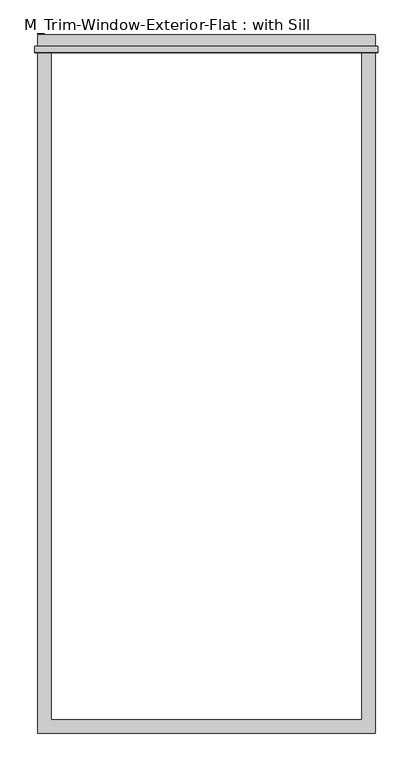
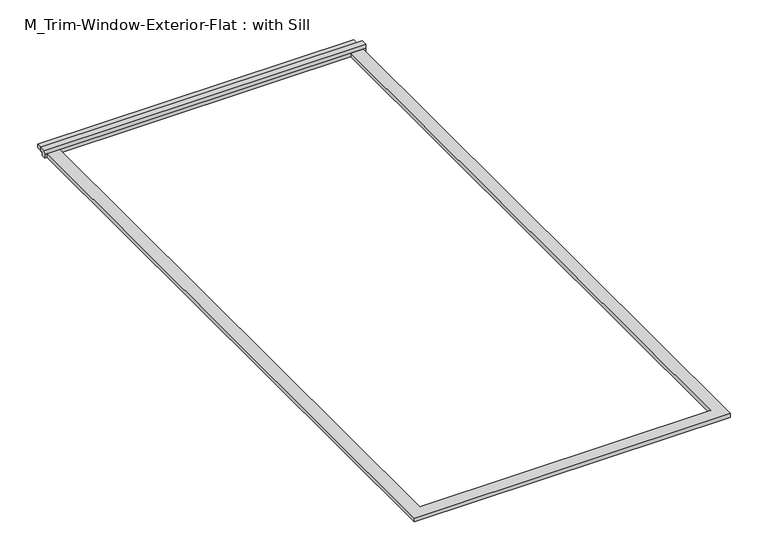
"""IFC4 building model written with IfcOpenShell, lengths in millimetres: proxy geometry, M_Trim-Window-Exterior-Flat : with Sill."""

import ifcopenshell
import ifcopenshell.guid

model = None  # the IFC model being written
_history = None  # IfcOwnerHistory: only IFC2X3 demands one
_inside = {}  # id of a spatial element -> (the spatial element, [elements in it])
_under = {}  # id of a project, library or spatial element -> (it, [spatial elements below it])
_declared = {}  # id of a project -> (the project, [libraries it declares])
_typed = {}  # id of a type object -> (the type object, [elements of that type])
_made_of = {}  # id of a material, layer set ... -> (it, [elements and type objects made of it])


def new_model(schema):
    """Start an empty IFC model of exactly this schema.

    Asked for "IFC4X3", IfcOpenShell would pick the latest addendum, in which some entities
    have other attributes; the version numbers below select the first issue.
    IFC2X3 requires an IfcOwnerHistory on every rooted entity: one is made here for all.
    """
    global model, _history
    if schema == "IFC4X3":
        model = ifcopenshell.file(schema_version=(4, 3, 0, 0))
    else:
        model = ifcopenshell.file(schema=schema)
    _inside.clear()
    _under.clear()
    _declared.clear()
    _typed.clear()
    _made_of.clear()
    _history = None
    if model.schema == "IFC2X3":
        org = make("IfcOrganization", Name="unknown")
        user = make(
            "IfcPersonAndOrganization",
            ThePerson=make("IfcPerson", FamilyName="unknown"),
            TheOrganization=org,
        )
        app = make(
            "IfcApplication",
            ApplicationDeveloper=org,
            Version="unknown",
            ApplicationFullName="unknown",
            ApplicationIdentifier="unknown",
        )
        _history = make(
            "IfcOwnerHistory",
            OwningUser=user,
            OwningApplication=app,
            ChangeAction="ADDED",
            CreationDate=0,
        )
    return model


def make(cls, **values):
    """One entity of the class cls with the attributes given. An attribute that is None is left unset."""
    return model.create_entity(
        cls, **{name: value for name, value in values.items() if value is not None}
    )


def rooted(cls, **values):
    """An entity with a GlobalId (a new one), such as an element, a storey or a relation."""
    return make(cls, GlobalId=ifcopenshell.guid.new(), OwnerHistory=_history, **values)


def si_unit(unit_type, name, prefix=None):
    """IfcSIUnit, for example si_unit("LENGTHUNIT", "METRE", prefix="MILLI")."""
    return make("IfcSIUnit", UnitType=unit_type, Prefix=prefix, Name=name)


def assignment(units):
    """IfcUnitAssignment: the units of a project."""
    return None if units is None else make("IfcUnitAssignment", Units=units)


def point(xyz):
    """IfcCartesianPoint."""
    return None if xyz is None else make("IfcCartesianPoint", Coordinates=xyz)


def direction(xyz):
    """IfcDirection."""
    return None if xyz is None else make("IfcDirection", DirectionRatios=xyz)


def frame(location, z_axis=None, x_axis=None):
    """IfcAxis2Placement3D, a coordinate frame: its origin and axes. An axis left out is left unset."""
    return make(
        "IfcAxis2Placement3D",
        Location=point(location),
        Axis=direction(z_axis),
        RefDirection=direction(x_axis),
    )


def origin():
    """The frame at (0, 0, 0) with its axes left unset."""
    return frame((0.0, 0.0, 0.0))


def origin_with_axes():
    """The frame at (0, 0, 0) with the z axis (0, 0, 1) and the x axis (1, 0, 0) written out."""
    return frame((0.0, 0.0, 0.0), z_axis=(0.0, 0.0, 1.0), x_axis=(1.0, 0.0, 0.0))


def place(relative_to, where):
    """IfcLocalPlacement: puts the frame where relative to a parent placement (None: the world)."""
    return make(
        "IfcLocalPlacement", PlacementRelTo=relative_to, RelativePlacement=where
    )


def context(
    kind, dimensions, precision=None, world=None, true_north=None, identifier=None
):
    """IfcGeometricRepresentationContext, for example the 3D "Model" context."""
    return make(
        "IfcGeometricRepresentationContext",
        ContextIdentifier=identifier,
        ContextType=kind,
        CoordinateSpaceDimension=dimensions,
        Precision=precision,
        WorldCoordinateSystem=world,
        TrueNorth=true_north,
    )


def project(units=None, contexts=None):
    """IfcProject with its units and contexts."""
    return rooted(
        "IfcProject",
        Name="project",
        RepresentationContexts=contexts,
        UnitsInContext=assignment(units),
    )


def spatial(cls, under=None, at=None, **own):
    """A site, building, storey or space (cls), placed at a placement, below another one or the project."""
    s = rooted(cls, ObjectPlacement=at, **own)
    if under is not None:
        _under.setdefault(under.id(), (under, []))[1].append(s)
    return s


def polyline(points):
    """IfcPolyline through the points."""
    return make("IfcPolyline", Points=[point(p) for p in points])


def outline(outer, holes=None, kind="AREA"):
    """IfcArbitraryClosedProfileDef: a profile drawn as a closed curve; with holes, ...WithVoids."""
    if holes is None:
        return make("IfcArbitraryClosedProfileDef", ProfileType=kind, OuterCurve=outer)
    return make(
        "IfcArbitraryProfileDefWithVoids",
        ProfileType=kind,
        OuterCurve=outer,
        InnerCurves=holes,
    )


def extrude(swept, where, along, depth):
    """IfcExtrudedAreaSolid: the profile swept, set in the frame where, extruded along a direction by depth."""
    return make(
        "IfcExtrudedAreaSolid",
        SweptArea=swept,
        Position=where,
        ExtrudedDirection=direction(along),
        Depth=depth,
    )


def shape(context_of_items, identifier, shape_type, items):
    """IfcShapeRepresentation: the items that make up one representation, for example the "Body"."""
    return make(
        "IfcShapeRepresentation",
        ContextOfItems=context_of_items,
        RepresentationIdentifier=identifier,
        RepresentationType=shape_type,
        Items=items,
    )


def source(mapping_origin, context_of_items, identifier, shape_type, items):
    """IfcRepresentationMap: a shape defined once, which mapped items show again and again."""
    return make(
        "IfcRepresentationMap",
        MappingOrigin=mapping_origin,
        MappedRepresentation=shape(context_of_items, identifier, shape_type, items),
    )


def transform(
    local_origin,
    x_axis=None,
    y_axis=None,
    z_axis=None,
    scale=None,
    scale2=None,
    scale3=None,
    uniform=True,
):
    """IfcCartesianTransformationOperator3D, or its non-uniform kind. x_axis, y_axis, z_axis: its Axis1, 2, 3."""
    if uniform:
        return make(
            "IfcCartesianTransformationOperator3D",
            Axis1=direction(x_axis),
            Axis2=direction(y_axis),
            LocalOrigin=point(local_origin),
            Scale=scale,
            Axis3=direction(z_axis),
        )
    return make(
        "IfcCartesianTransformationOperator3DnonUniform",
        Axis1=direction(x_axis),
        Axis2=direction(y_axis),
        LocalOrigin=point(local_origin),
        Scale=scale,
        Axis3=direction(z_axis),
        Scale2=scale2,
        Scale3=scale3,
    )


def mapped(mapping_source, mapping_target):
    """IfcMappedItem: shows the shape of a source again, moved by a transform."""
    return make(
        "IfcMappedItem", MappingSource=mapping_source, MappingTarget=mapping_target
    )


def made_of(thing, what):
    """Note that an element or type object is made of a material, layer set ...; save() writes the relation."""
    if what is not None:
        _made_of.setdefault(what.id(), (what, []))[1].append(thing)
    return thing


def element(
    cls,
    number,
    at=None,
    inside=None,
    cuts=None,
    type_object=None,
    material=None,
    context=None,
    identifier="Body",
    shape_type=None,
    held_by="IfcProductDefinitionShape",
    body=None,
    shapes=None,
    **own,
):
    """One element of the class cls, such as IfcWall. Its Tag is "e" and its number.

    at: its placement. inside: the storey or other place that contains it. cuts: it is an
    opening in that element (IfcRelVoidsElement). A single representation is given by context,
    identifier, shape_type and body (its items); several are given by shapes. held_by: the class
    of the entity that holds the representations. save() writes the other relations.
    """
    e = rooted(cls, Tag="e%d" % number, ObjectPlacement=at, **own)
    if body is not None:
        shapes = [shape(context, identifier, shape_type, body)]
    if shapes is not None:
        e.Representation = make(held_by, Representations=shapes)
    if inside is not None:
        _inside.setdefault(inside.id(), (inside, []))[1].append(e)
    if cuts is not None:
        rooted(
            "IfcRelVoidsElement", RelatingBuildingElement=cuts, RelatedOpeningElement=e
        )
    if type_object is not None:
        _typed.setdefault(type_object.id(), (type_object, []))[1].append(e)
    return made_of(e, material)


def aggregate(whole, parts):
    """IfcRelAggregates: a whole, such as a stair, and the parts it consists of."""
    return rooted("IfcRelAggregates", RelatingObject=whole, RelatedObjects=parts)


def save(model, path):
    """Write the relations noted so far, then the file.

    IfcRelAggregates (storeys below a building ...), IfcRelContainedInSpatialStructure (elements
    in a storey), IfcRelDefinesByType, IfcRelAssociatesMaterial and IfcRelDeclares: one each for
    every whole, place, type object, material and project.
    """
    for whole, parts in _under.values():
        aggregate(whole, parts)
    for where, things in _inside.values():
        rooted(
            "IfcRelContainedInSpatialStructure",
            RelatedElements=things,
            RelatingStructure=where,
        )
    for kind, things in _typed.values():
        rooted("IfcRelDefinesByType", RelatedObjects=things, RelatingType=kind)
    for what, things in _made_of.values():
        rooted("IfcRelAssociatesMaterial", RelatedObjects=things, RelatingMaterial=what)
    for by, libraries in _declared.values():
        rooted("IfcRelDeclares", RelatingContext=by, RelatedDefinitions=libraries)
    model.write(path)


def m_trim_window_exterior_flat_with_sill_53234c90(model_context):
    return source(origin(), model_context, "Body", "SweptSolid", [
        extrude(outline(polyline([(760.0, 3020.4323709), (-760.0, 3020.4323709), (-760.0, 3080.4323709), (760.0, 3080.4323709), (760.0, 3020.4323709)])), origin_with_axes(), (0.0, 0.0, 1.0), 19.05),
        extrude(outline(polyline([(3030.0, 38.1), (3030.0, 19.05), (3020.4323709, 19.05), (3020.4323709, 0.0), (3000.0, 0.0), (3000.0, 19.05), (3002.4580645, 38.1), (3030.0, 38.1)])), frame((-772.7, 0.0, 0.0), z_axis=(1.0, 0.0, 0.0), x_axis=(0.0, 1.0, 0.0)), (0.0, 0.0, 1.0), 1545.4),
        extrude(outline(polyline([(-760.0, -60.0), (-760.0, 3000.0), (-700.0, 3000.0), (-700.0, 0.0), (700.0, 0.0), (700.0, 3000.0), (760.0, 3000.0), (760.0, -60.0), (-760.0, -60.0)])), origin_with_axes(), (0.0, 0.0, 1.0), 19.05),
    ])


if __name__ == "__main__":
    model = new_model("IFC4")
    model_context = context("Model", 3, world=origin())
    ifc_project = project(units=[si_unit("LENGTHUNIT", "METRE", prefix="MILLI")], contexts=[model_context])
    site = spatial("IfcSite", under=ifc_project)
    building = spatial("IfcBuilding", under=site)
    placement = place(None, origin())
    m_trim_window_exterior_flat_with_sill_shape = m_trim_window_exterior_flat_with_sill_53234c90(model_context)
    element("IfcBuildingElementProxy", 1, Name="M_Trim-Window-Exterior-Flat : with Sill", ObjectType="M_Trim-Window-Exterior-Flat : with Sill", at=placement, inside=building, context=model_context, shape_type="MappedRepresentation", body=[
        mapped(m_trim_window_exterior_flat_with_sill_shape, transform((0.0, 0.0, 0.0), x_axis=(1.0, 0.0, 0.0), y_axis=(0.0, 1.0, 0.0), z_axis=(0.0, 0.0, 1.0))),
    ])
    save(model, "model.ifc")

# Revit data of these elements
# Type "M_Trim-Window-Exterior-Flat : with Sill"
#   Trim Width = 60 mm
#   Trim Thickness_Picture Frame = 30 mm
#   Trim Thickness_with Sill = 19.05 mm
#   Sill Thickness = 30 mm
#   Opening Width [instance default] = 600 mm
#   Opening Height [instance default] = 900 mm
#   Default Elevation = 1200 mm
#   Sill = yes
#   Picture Frame = no
#   Trim Material [instance default] = none
# Element 1 (IfcBuildingElementProxy, "M_Trim-Window-Exterior-Flat : with Sill")
#   Opening Width = 1400 mm
#   Opening Height = 3000 mm
#   Trim Material = Clad - White
#   Materials on its faces: "Clad - White"
# Materials
#   "Clad - White": class "Wood", colour RGB 245 245 243, transparency 0, Cost = 0
